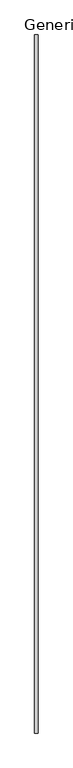
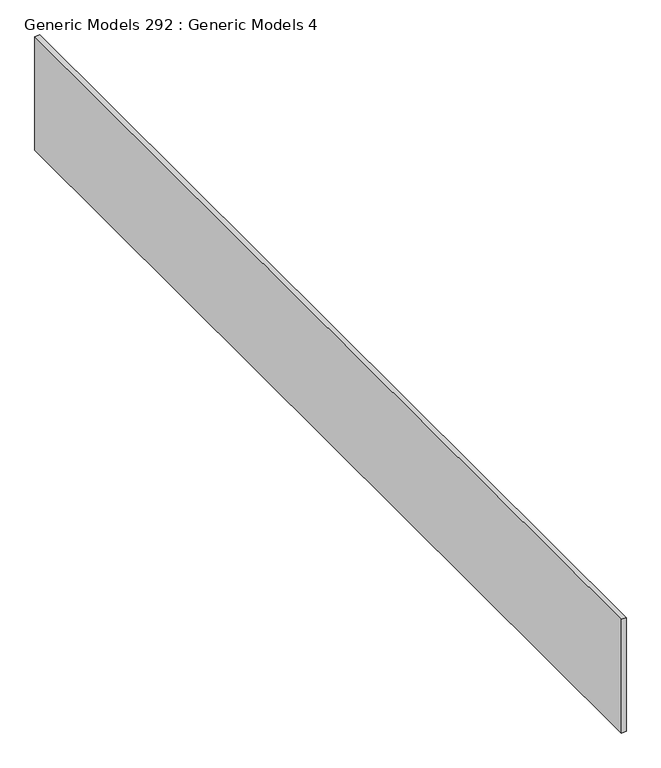
"""IFC4 building model written with IfcOpenShell, lengths in millimetres: proxy geometry, Generic Models 292 : Generic Models 4."""

from ifc_helpers import new_model, si_unit, frame, origin, place, context, project, spatial, polyline, outline, extrude, source, transform, mapped, element, save


def generic_models_292_generic_models_4_fae2383a(model_context):
    return source(origin(), model_context, "Body", "SweptSolid", [
        extrude(outline(polyline([(7253.8514146, 7765.4769662), (7234.8014146, 7765.4769662), (7234.8014146, 11778.6769662), (7253.8514146, 11778.6769662), (7253.8514146, 7765.4769662)])), frame((0.0, 0.0, 126809.341198), z_axis=(0.0, 0.0, 1.0), x_axis=(1.0, 0.0, 0.0)), (0.0, 0.0, 1.0), 474.3603487),
    ])


if __name__ == "__main__":
    model = new_model("IFC4")
    model_context = context("Model", 3, world=origin())
    ifc_project = project(units=[si_unit("LENGTHUNIT", "METRE", prefix="MILLI")], contexts=[model_context])
    site = spatial("IfcSite", under=ifc_project)
    building = spatial("IfcBuilding", under=site)
    placement = place(None, origin())
    generic_models_292_generic_models_4_shape = generic_models_292_generic_models_4_fae2383a(model_context)
    element("IfcBuildingElementProxy", 1, Name="Generic Models 292 : Generic Models 4", ObjectType="Generic Models 292 : Generic Models 4", at=placement, inside=building, context=model_context, shape_type="MappedRepresentation", body=[
        mapped(generic_models_292_generic_models_4_shape, transform((0.0, 0.0, 0.0), x_axis=(1.0, 0.0, 0.0), y_axis=(0.0, 1.0, 0.0), z_axis=(0.0, 0.0, 1.0))),
    ])
    save(model, "model.ifc")

# Revit data of these elements
# Element 1 (IfcBuildingElementProxy, "Generic Models 292 : Generic Models 4")
#   Materials on its faces: "_CDX PLYWOOD - SEE STRUCT DWGs"
# Materials
#   "_CDX PLYWOOD - SEE STRUCT DWGs": class "Generic", colour RGB 98 75 74, transparency 0, Cost = 0
